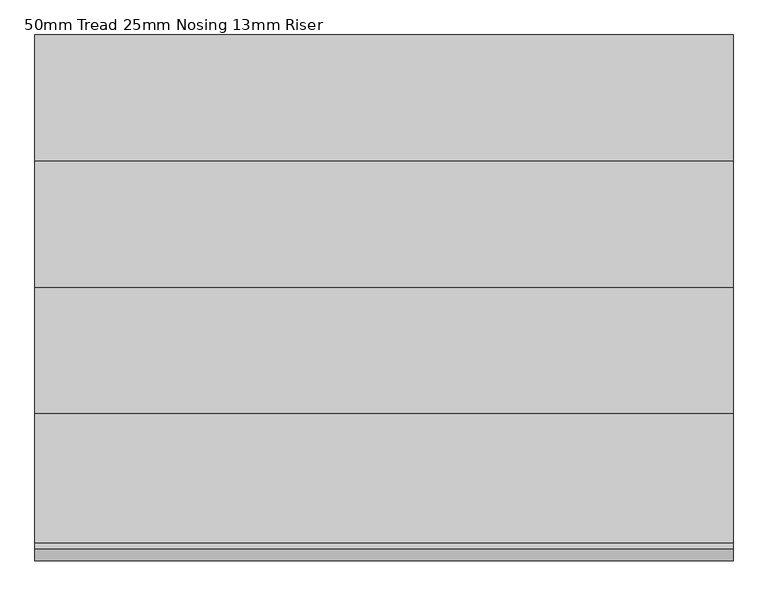
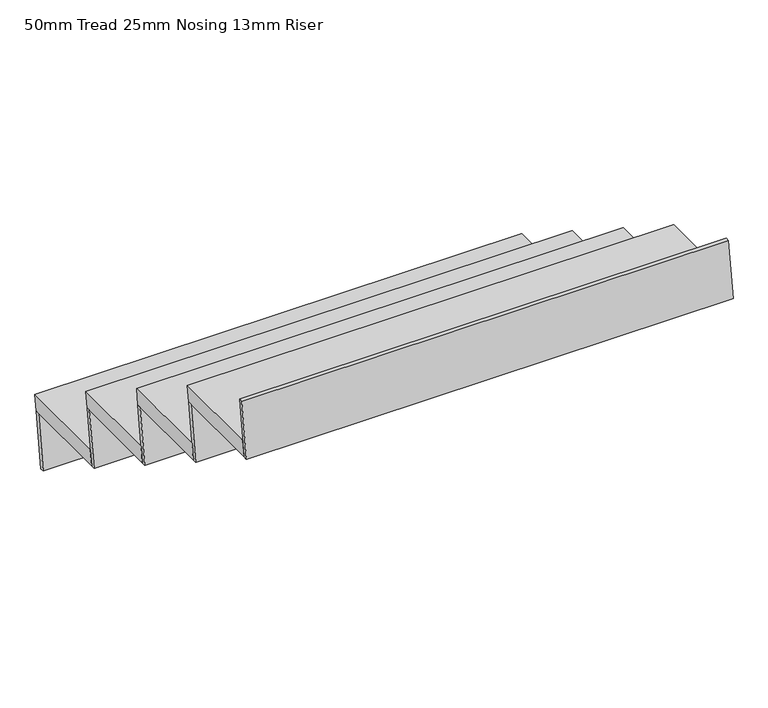
"""IFC4 building model written with IfcOpenShell, lengths in millimetres: stair flight geometry, 50mm Tread 25mm Nosing 13mm Riser."""

from ifc_helpers import new_model, si_unit, frame, origin, place, context, project, spatial, polyline, outline, extrude, source, transform, mapped, element, save


def stair_flight_50mm_tread_25mm_nosing_13mm_riser_c8de7c0f(model_context):
    return source(origin(), model_context, "Body", "SweptSolid", [
        extrude(outline(polyline([(7032.4781803, 11794.1176471), (7332.4781803, 11794.1176471), (7325.3948469, 11744.1176471), (7025.3948469, 11744.1176471), (7032.4781803, 11794.1176471)])), frame((-226.7120949, 0.0, 0.0), z_axis=(1.0, 0.0, 0.0), x_axis=(0.0, 1.0, 0.0)), (0.0, 0.0, 1.0), 1520.0),
        extrude(outline(polyline([(7325.3948469, 11744.1176471), (7300.3948469, 11567.6470588), (7287.770036, 11567.6470588), (7312.770036, 11744.1176471), (7325.3948469, 11744.1176471)])), frame((-226.7120949, 0.0, 0.0), z_axis=(1.0, 0.0, 0.0), x_axis=(0.0, 1.0, 0.0)), (0.0, 0.0, 1.0), 1520.0),
        extrude(outline(polyline([(7050.3948469, 11920.5882353), (7025.3948469, 11744.1176471), (7012.770036, 11744.1176471), (7037.770036, 11920.5882353), (7050.3948469, 11920.5882353)])), frame((-226.7120949, 0.0, 0.0), z_axis=(1.0, 0.0, 0.0), x_axis=(0.0, 1.0, 0.0)), (0.0, 0.0, 1.0), 1520.0),
        extrude(outline(polyline([(6757.4781803, 11970.5882353), (7057.4781803, 11970.5882353), (7050.3948469, 11920.5882353), (6750.3948469, 11920.5882353), (6757.4781803, 11970.5882353)])), frame((-226.7120949, 0.0, 0.0), z_axis=(1.0, 0.0, 0.0), x_axis=(0.0, 1.0, 0.0)), (0.0, 0.0, 1.0), 1520.0),
        extrude(outline(polyline([(6775.3948469, 12097.0588235), (6750.3948469, 11920.5882353), (6737.770036, 11920.5882353), (6762.770036, 12097.0588235), (6775.3948469, 12097.0588235)])), frame((-226.7120949, 0.0, 0.0), z_axis=(1.0, 0.0, 0.0), x_axis=(0.0, 1.0, 0.0)), (0.0, 0.0, 1.0), 1520.0),
        extrude(outline(polyline([(6482.4781803, 12147.0588235), (6782.4781803, 12147.0588235), (6775.3948469, 12097.0588235), (6475.3948469, 12097.0588235), (6482.4781803, 12147.0588235)])), frame((-226.7120949, 0.0, 0.0), z_axis=(1.0, 0.0, 0.0), x_axis=(0.0, 1.0, 0.0)), (0.0, 0.0, 1.0), 1520.0),
        extrude(outline(polyline([(6500.3948469, 12273.5294118), (6475.3948469, 12097.0588235), (6462.770036, 12097.0588235), (6487.770036, 12273.5294118), (6500.3948469, 12273.5294118)])), frame((-226.7120949, 0.0, 0.0), z_axis=(1.0, 0.0, 0.0), x_axis=(0.0, 1.0, 0.0)), (0.0, 0.0, 1.0), 1520.0),
        extrude(outline(polyline([(6225.3948469, 12450.0), (6200.3948469, 12273.5294118), (6187.770036, 12273.5294118), (6212.770036, 12450.0), (6225.3948469, 12450.0)])), frame((-226.7120949, 0.0, 0.0), z_axis=(1.0, 0.0, 0.0), x_axis=(0.0, 1.0, 0.0)), (0.0, 0.0, 1.0), 1520.0),
        extrude(outline(polyline([(6207.4781803, 12323.5294118), (6507.4781803, 12323.5294118), (6500.3948469, 12273.5294118), (6200.3948469, 12273.5294118), (6207.4781803, 12323.5294118)])), frame((-226.7120949, 0.0, 0.0), z_axis=(1.0, 0.0, 0.0), x_axis=(0.0, 1.0, 0.0)), (0.0, 0.0, 1.0), 1520.0),
    ])


if __name__ == "__main__":
    model = new_model("IFC4")
    model_context = context("Model", 3, world=origin())
    ifc_project = project(units=[si_unit("LENGTHUNIT", "METRE", prefix="MILLI")], contexts=[model_context])
    site = spatial("IfcSite", under=ifc_project)
    building = spatial("IfcBuilding", under=site)
    placement = place(None, origin())
    stair_flight_50mm_tread_25mm_nosing_13mm_riser_shape = stair_flight_50mm_tread_25mm_nosing_13mm_riser_c8de7c0f(model_context)
    element("IfcStairFlight", 1, ObjectType="50mm Tread 25mm Nosing 13mm Riser", at=placement, inside=building, context=model_context, shape_type="MappedRepresentation", body=[
        mapped(stair_flight_50mm_tread_25mm_nosing_13mm_riser_shape, transform((0.0, 0.0, 0.0), x_axis=(1.0, 0.0, 0.0), y_axis=(0.0, 1.0, 0.0), z_axis=(0.0, 0.0, 1.0))),
    ])
    save(model, "model.ifc")
